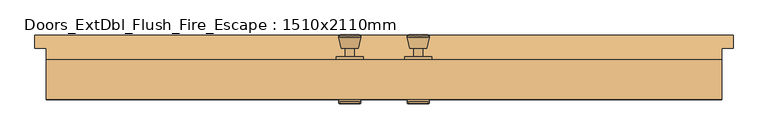
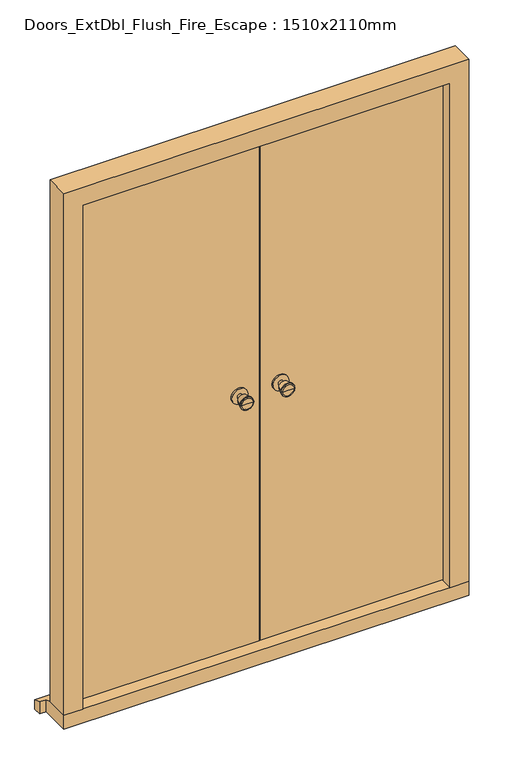
"""IFC4 building model written with IfcOpenShell, lengths in millimetres: door geometry, Doors_ExtDbl_Flush_Fire_Escape : 1510x2110mm."""

from ifc_helpers import new_model, si_unit, point, frame, frame_2d, origin, place, context, project, spatial, polyline, circle_curve, trimmed, segment, composite_curve, outline, extrude, faceted_brep, source, transform, mapped, element, save
from ifc_brep_helpers import plane_surface, cylinder_surface, revolved_surface, advanced_brep


def doors_extdbl_flush_fire_escape_1510x2110mm_f48bbf68(model_context):
    return source(origin(), model_context, "Body", "SolidModel", [
        advanced_brep(
        [(-76.5, 156.0, 1050.0), (-86.5, 156.0, 1050.0), (-66.5, 156.0, 1050.0), (-96.9758676, 205.0, 1050.0), (-76.5, 205.0, 1050.0), (-56.0241324, 205.0, 1050.0), (-101.5, 203.1721319, 1050.0), (-51.5, 203.1721319, 1050.0), (-101.5, 199.7084537, 1050.0), (-51.5, 199.7084537, 1050.0), (-95.136236, 175.0, 1050.0), (-57.863764, 175.0, 1050.0), (-86.5, 175.0, 1050.0), (-66.5, 175.0, 1050.0)],
        [
            (0, 1),
            (1, 2, circle_curve(frame((-76.5, 156.0, 1050.0), z_axis=(0.0, -1.0, 0.0), x_axis=(1.0, 0.0, 0.0)), 10.0)),
            (2, 0),
            (2, 1, circle_curve(frame((-76.5, 156.0, 1050.0), z_axis=(0.0, -1.0, 0.0), x_axis=(1.0, 0.0, 0.0)), 10.0)),
            (3, 4),
            (4, 5),
            (5, 3, circle_curve(frame((-76.5, 205.0, 1050.0), z_axis=(0.0, 1.0, 0.0), x_axis=(1.0, 0.0, 0.0)), 20.4758676)),
            (3, 5, circle_curve(frame((-76.5, 205.0, 1050.0), z_axis=(0.0, 1.0, 0.0), x_axis=(1.0, 0.0, 0.0)), 20.4758676)),
            (6, 3),
            (5, 7),
            (7, 6, circle_curve(frame((-76.5, 203.1721319, 1050.0), z_axis=(0.0, 1.0, 0.0), x_axis=(1.0, 0.0, 0.0)), 25.0)),
            (6, 7, circle_curve(frame((-76.5, 203.1721319, 1050.0), z_axis=(0.0, 1.0, 0.0), x_axis=(1.0, 0.0, 0.0)), 25.0)),
            (8, 6),
            (7, 9),
            (9, 8, circle_curve(frame((-76.5, 199.7084537, 1050.0), z_axis=(0.0, 1.0, 0.0), x_axis=(1.0, 0.0, 0.0)), 25.0)),
            (8, 9, circle_curve(frame((-76.5, 199.7084537, 1050.0), z_axis=(0.0, 1.0, 0.0), x_axis=(1.0, 0.0, 0.0)), 25.0)),
            (10, 8),
            (9, 11),
            (11, 10, circle_curve(frame((-76.5, 175.0, 1050.0), z_axis=(0.0, 1.0, 0.0), x_axis=(1.0, 0.0, 0.0)), 18.636236)),
            (10, 11, circle_curve(frame((-76.5, 175.0, 1050.0), z_axis=(0.0, 1.0, 0.0), x_axis=(1.0, 0.0, 0.0)), 18.636236)),
            (12, 10),
            (11, 13),
            (13, 12, circle_curve(frame((-76.5, 175.0, 1050.0), z_axis=(0.0, 1.0, 0.0), x_axis=(1.0, 0.0, 0.0)), 10.0)),
            (12, 13, circle_curve(frame((-76.5, 175.0, 1050.0), z_axis=(0.0, 1.0, 0.0), x_axis=(1.0, 0.0, 0.0)), 10.0)),
            (1, 12),
            (13, 2),
        ],
        [
            plane_surface(frame((-76.5, 156.0, 1050.0), z_axis=(0.0, -1.0, 0.0), x_axis=(1.0, 0.0, 0.0))),
            plane_surface(frame((-76.5, 205.0, 1050.0), z_axis=(0.0, 1.0, 0.0), x_axis=(1.0, 0.0, 0.0))),
            revolved_surface(polyline([(-56.0241324, 205.0, 1050.0), (-51.5, 203.1721319, 1050.0)]), (-76.5, 156.0, 1050.0), (0.0, -1.0, 0.0)),
            cylinder_surface(frame((-76.5, 156.0, 1050.0), z_axis=(0.0, -1.0, 0.0), x_axis=(1.0, 0.0, 0.0)), 25.0),
            revolved_surface(polyline([(-51.5, 199.7084537, 1050.0), (-57.863764, 175.0, 1050.0)]), (-76.5, 156.0, 1050.0), (0.0, -1.0, 0.0)),
            plane_surface(frame((-76.5, 175.0, 1050.0), z_axis=(0.0, -1.0, 0.0), x_axis=(1.0, 0.0, 0.0))),
            cylinder_surface(frame((-76.5, 156.0, 1050.0), z_axis=(0.0, -1.0, 0.0), x_axis=(1.0, 0.0, 0.0)), 10.0),
        ],
        [
            (0, [[1, 2, 3]]),
            (0, [[-3, 4, -1]]),
            (1, [[5, 6, 7]]),
            (1, [[-6, -5, 8]]),
            (2, [[9, -7, 10, 11]]),
            (2, [[-10, -8, -9, 12]]),
            (3, [[13, -11, 14, 15]]),
            (3, [[-14, -12, -13, 16]]),
            (4, [[17, -15, 18, 19]]),
            (4, [[-18, -16, -17, 20]]),
            (5, [[21, -19, 22, 23]]),
            (5, [[-22, -20, -21, 24]]),
            (6, [[25, -23, 26, -2]]),
            (6, [[-26, -24, -25, -4]]),
        ],
    ),
        extrude(outline(composite_curve([segment(trimmed(circle_curve(frame_2d((1050.0, -76.5)), 30.0), [point((1050.0, -46.5))], [point((1050.0, -106.5))], False, "CARTESIAN"), True, "CONTINUOUS"), segment(trimmed(circle_curve(frame_2d((1050.0, -76.5)), 30.0), [point((1050.0, -106.5))], [point((1050.0, -46.5))], False, "CARTESIAN"), True, "CONTINUOUS")], self_intersect=False)), frame((0.0, 150.0, 0.0), z_axis=(0.0, 1.0, 0.0), x_axis=(0.0, 0.0, 1.0)), (0.0, 0.0, 1.0), 6.0),
        advanced_brep(
        [(-76.5, 100.0, 1050.0), (-66.5, 100.0, 1050.0), (-86.5, 100.0, 1050.0), (-96.9758676, 51.0, 1050.0), (-56.0241324, 51.0, 1050.0), (-76.5, 51.0, 1050.0), (-101.5, 52.8278681, 1050.0), (-51.5, 52.8278681, 1050.0), (-101.5, 56.2915463, 1050.0), (-51.5, 56.2915463, 1050.0), (-95.136236, 81.0, 1050.0), (-57.863764, 81.0, 1050.0), (-86.5, 81.0, 1050.0), (-66.5, 81.0, 1050.0)],
        [
            (0, 1),
            (1, 2, circle_curve(frame((-76.5, 100.0, 1050.0), z_axis=(0.0, 1.0, 0.0), x_axis=(1.0, 0.0, 0.0)), 10.0)),
            (2, 0),
            (2, 1, circle_curve(frame((-76.5, 100.0, 1050.0), z_axis=(0.0, 1.0, 0.0), x_axis=(1.0, 0.0, 0.0)), 10.0)),
            (3, 4, circle_curve(frame((-76.5, 51.0, 1050.0), z_axis=(0.0, -1.0, 0.0), x_axis=(1.0, 0.0, 0.0)), 20.4758676)),
            (4, 5),
            (5, 3),
            (4, 3, circle_curve(frame((-76.5, 51.0, 1050.0), z_axis=(0.0, -1.0, 0.0), x_axis=(1.0, 0.0, 0.0)), 20.4758676)),
            (6, 7, circle_curve(frame((-76.5, 52.8278681, 1050.0), z_axis=(0.0, -1.0, 0.0), x_axis=(1.0, 0.0, 0.0)), 25.0)),
            (7, 4),
            (3, 6),
            (7, 6, circle_curve(frame((-76.5, 52.8278681, 1050.0), z_axis=(0.0, -1.0, 0.0), x_axis=(1.0, 0.0, 0.0)), 25.0)),
            (8, 9, circle_curve(frame((-76.5, 56.2915463, 1050.0), z_axis=(0.0, -1.0, 0.0), x_axis=(1.0, 0.0, 0.0)), 25.0)),
            (9, 7),
            (6, 8),
            (9, 8, circle_curve(frame((-76.5, 56.2915463, 1050.0), z_axis=(0.0, -1.0, 0.0), x_axis=(1.0, 0.0, 0.0)), 25.0)),
            (10, 11, circle_curve(frame((-76.5, 81.0, 1050.0), z_axis=(0.0, -1.0, 0.0), x_axis=(1.0, 0.0, 0.0)), 18.636236)),
            (11, 9),
            (8, 10),
            (11, 10, circle_curve(frame((-76.5, 81.0, 1050.0), z_axis=(0.0, -1.0, 0.0), x_axis=(1.0, 0.0, 0.0)), 18.636236)),
            (12, 13, circle_curve(frame((-76.5, 81.0, 1050.0), z_axis=(0.0, -1.0, 0.0), x_axis=(1.0, 0.0, 0.0)), 10.0)),
            (13, 11),
            (10, 12),
            (13, 12, circle_curve(frame((-76.5, 81.0, 1050.0), z_axis=(0.0, -1.0, 0.0), x_axis=(1.0, 0.0, 0.0)), 10.0)),
            (1, 13),
            (12, 2),
        ],
        [
            plane_surface(frame((-76.5, 100.0, 1050.0), z_axis=(0.0, 1.0, 0.0), x_axis=(1.0, 0.0, 0.0))),
            plane_surface(frame((-76.5, 51.0, 1050.0), z_axis=(0.0, -1.0, 0.0), x_axis=(1.0, 0.0, 0.0))),
            revolved_surface(polyline([(-56.0241324, 51.0, 1050.0), (-51.5, 52.8278681, 1050.0)]), (-76.5, 100.0, 1050.0), (0.0, 1.0, 0.0)),
            cylinder_surface(frame((-76.5, 100.0, 1050.0), z_axis=(0.0, 1.0, 0.0), x_axis=(1.0, 0.0, 0.0)), 25.0),
            revolved_surface(polyline([(-51.5, 56.2915463, 1050.0), (-57.863764, 81.0, 1050.0)]), (-76.5, 100.0, 1050.0), (0.0, 1.0, 0.0)),
            plane_surface(frame((-76.5, 81.0, 1050.0), z_axis=(0.0, 1.0, 0.0), x_axis=(1.0, 0.0, 0.0))),
            cylinder_surface(frame((-76.5, 100.0, 1050.0), z_axis=(0.0, 1.0, 0.0), x_axis=(1.0, 0.0, 0.0)), 10.0),
        ],
        [
            (0, [[1, 2, 3]]),
            (0, [[-3, 4, -1]]),
            (1, [[5, 6, 7]]),
            (1, [[8, -7, -6]]),
            (2, [[9, 10, -5, 11]]),
            (2, [[12, -11, -8, -10]]),
            (3, [[13, 14, -9, 15]]),
            (3, [[16, -15, -12, -14]]),
            (4, [[17, 18, -13, 19]]),
            (4, [[20, -19, -16, -18]]),
            (5, [[21, 22, -17, 23]]),
            (5, [[24, -23, -20, -22]]),
            (6, [[-2, 25, -21, 26]]),
            (6, [[-4, -26, -24, -25]]),
        ],
    ),
        extrude(outline(composite_curve([segment(trimmed(circle_curve(frame_2d((1050.0, -76.5)), 30.0), [point((1050.0, -46.5))], [point((1050.0, -106.5))], False, "CARTESIAN"), True, "CONTINUOUS"), segment(trimmed(circle_curve(frame_2d((1050.0, -76.5)), 30.0), [point((1050.0, -106.5))], [point((1050.0, -46.5))], False, "CARTESIAN"), True, "CONTINUOUS")], self_intersect=False)), frame((0.0, 100.0, 0.0), z_axis=(0.0, 1.0, 0.0), x_axis=(0.0, 0.0, 1.0)), (0.0, 0.0, 1.0), 6.0),
        advanced_brep(
        [(76.5, 156.0, 1050.0), (66.5, 156.0, 1050.0), (86.5, 156.0, 1050.0), (96.9758676, 205.0, 1050.0), (56.0241324, 205.0, 1050.0), (76.5, 205.0, 1050.0), (101.5, 203.1721319, 1050.0), (51.5, 203.1721319, 1050.0), (101.5, 199.7084537, 1050.0), (51.5, 199.7084537, 1050.0), (95.136236, 175.0, 1050.0), (57.863764, 175.0, 1050.0), (86.5, 175.0, 1050.0), (66.5, 175.0, 1050.0)],
        [
            (0, 1),
            (1, 2, circle_curve(frame((76.5, 156.0, 1050.0), z_axis=(0.0, -1.0, 0.0), x_axis=(-1.0, 0.0, 0.0)), 10.0)),
            (2, 0),
            (2, 1, circle_curve(frame((76.5, 156.0, 1050.0), z_axis=(0.0, -1.0, 0.0), x_axis=(-1.0, 0.0, 0.0)), 10.0)),
            (3, 4, circle_curve(frame((76.5, 205.0, 1050.0), z_axis=(0.0, 1.0, 0.0), x_axis=(-1.0, 0.0, 0.0)), 20.4758676)),
            (4, 5),
            (5, 3),
            (4, 3, circle_curve(frame((76.5, 205.0, 1050.0), z_axis=(0.0, 1.0, 0.0), x_axis=(-1.0, 0.0, 0.0)), 20.4758676)),
            (6, 7, circle_curve(frame((76.5, 203.1721319, 1050.0), z_axis=(0.0, 1.0, 0.0), x_axis=(-1.0, 0.0, 0.0)), 25.0)),
            (7, 4),
            (3, 6),
            (7, 6, circle_curve(frame((76.5, 203.1721319, 1050.0), z_axis=(0.0, 1.0, 0.0), x_axis=(-1.0, 0.0, 0.0)), 25.0)),
            (8, 9, circle_curve(frame((76.5, 199.7084537, 1050.0), z_axis=(0.0, 1.0, 0.0), x_axis=(-1.0, 0.0, 0.0)), 25.0)),
            (9, 7),
            (6, 8),
            (9, 8, circle_curve(frame((76.5, 199.7084537, 1050.0), z_axis=(0.0, 1.0, 0.0), x_axis=(-1.0, 0.0, 0.0)), 25.0)),
            (10, 11, circle_curve(frame((76.5, 175.0, 1050.0), z_axis=(0.0, 1.0, 0.0), x_axis=(-1.0, 0.0, 0.0)), 18.636236)),
            (11, 9),
            (8, 10),
            (11, 10, circle_curve(frame((76.5, 175.0, 1050.0), z_axis=(0.0, 1.0, 0.0), x_axis=(-1.0, 0.0, 0.0)), 18.636236)),
            (12, 13, circle_curve(frame((76.5, 175.0, 1050.0), z_axis=(0.0, 1.0, 0.0), x_axis=(-1.0, 0.0, 0.0)), 10.0)),
            (13, 11),
            (10, 12),
            (13, 12, circle_curve(frame((76.5, 175.0, 1050.0), z_axis=(0.0, 1.0, 0.0), x_axis=(-1.0, 0.0, 0.0)), 10.0)),
            (1, 13),
            (12, 2),
        ],
        [
            plane_surface(frame((76.5, 156.0, 1050.0), z_axis=(0.0, -1.0, 0.0), x_axis=(-1.0, 0.0, 0.0))),
            plane_surface(frame((76.5, 205.0, 1050.0), z_axis=(0.0, 1.0, 0.0), x_axis=(-1.0, 0.0, 0.0))),
            revolved_surface(polyline([(56.0241324, 205.0, 1050.0), (51.5, 203.1721319, 1050.0)]), (76.5, 156.0, 1050.0), (0.0, -1.0, 0.0)),
            cylinder_surface(frame((76.5, 156.0, 1050.0), z_axis=(0.0, -1.0, 0.0), x_axis=(-1.0, 0.0, 0.0)), 25.0),
            revolved_surface(polyline([(51.5, 199.7084537, 1050.0), (57.863764, 175.0, 1050.0)]), (76.5, 156.0, 1050.0), (0.0, -1.0, 0.0)),
            plane_surface(frame((76.5, 175.0, 1050.0), z_axis=(0.0, -1.0, 0.0), x_axis=(-1.0, 0.0, 0.0))),
            cylinder_surface(frame((76.5, 156.0, 1050.0), z_axis=(0.0, -1.0, 0.0), x_axis=(-1.0, 0.0, 0.0)), 10.0),
        ],
        [
            (0, [[1, 2, 3]]),
            (0, [[-3, 4, -1]]),
            (1, [[5, 6, 7]]),
            (1, [[8, -7, -6]]),
            (2, [[9, 10, -5, 11]]),
            (2, [[12, -11, -8, -10]]),
            (3, [[13, 14, -9, 15]]),
            (3, [[16, -15, -12, -14]]),
            (4, [[17, 18, -13, 19]]),
            (4, [[20, -19, -16, -18]]),
            (5, [[21, 22, -17, 23]]),
            (5, [[24, -23, -20, -22]]),
            (6, [[-2, 25, -21, 26]]),
            (6, [[-4, -26, -24, -25]]),
        ],
    ),
        extrude(outline(composite_curve([segment(trimmed(circle_curve(frame_2d((1050.0, 76.5)), 30.0), [point((1050.0, 46.5))], [point((1050.0, 106.5))], False, "CARTESIAN"), True, "CONTINUOUS"), segment(trimmed(circle_curve(frame_2d((1050.0, 76.5)), 30.0), [point((1050.0, 106.5))], [point((1050.0, 46.5))], False, "CARTESIAN"), True, "CONTINUOUS")], self_intersect=False)), frame((0.0, 150.0, 0.0), z_axis=(0.0, 1.0, 0.0), x_axis=(0.0, 0.0, 1.0)), (0.0, 0.0, 1.0), 6.0),
        advanced_brep(
        [(76.5, 100.0, 1050.0), (86.5, 100.0, 1050.0), (66.5, 100.0, 1050.0), (96.9758676, 51.0, 1050.0), (76.5, 51.0, 1050.0), (56.0241324, 51.0, 1050.0), (101.5, 52.8278681, 1050.0), (51.5, 52.8278681, 1050.0), (101.5, 56.2915463, 1050.0), (51.5, 56.2915463, 1050.0), (95.136236, 81.0, 1050.0), (57.863764, 81.0, 1050.0), (86.5, 81.0, 1050.0), (66.5, 81.0, 1050.0)],
        [
            (0, 1),
            (1, 2, circle_curve(frame((76.5, 100.0, 1050.0), z_axis=(0.0, 1.0, 0.0), x_axis=(-1.0, 0.0, 0.0)), 10.0)),
            (2, 0),
            (2, 1, circle_curve(frame((76.5, 100.0, 1050.0), z_axis=(0.0, 1.0, 0.0), x_axis=(-1.0, 0.0, 0.0)), 10.0)),
            (3, 4),
            (4, 5),
            (5, 3, circle_curve(frame((76.5, 51.0, 1050.0), z_axis=(0.0, -1.0, 0.0), x_axis=(-1.0, 0.0, 0.0)), 20.4758676)),
            (3, 5, circle_curve(frame((76.5, 51.0, 1050.0), z_axis=(0.0, -1.0, 0.0), x_axis=(-1.0, 0.0, 0.0)), 20.4758676)),
            (6, 3),
            (5, 7),
            (7, 6, circle_curve(frame((76.5, 52.8278681, 1050.0), z_axis=(0.0, -1.0, 0.0), x_axis=(-1.0, 0.0, 0.0)), 25.0)),
            (6, 7, circle_curve(frame((76.5, 52.8278681, 1050.0), z_axis=(0.0, -1.0, 0.0), x_axis=(-1.0, 0.0, 0.0)), 25.0)),
            (8, 6),
            (7, 9),
            (9, 8, circle_curve(frame((76.5, 56.2915463, 1050.0), z_axis=(0.0, -1.0, 0.0), x_axis=(-1.0, 0.0, 0.0)), 25.0)),
            (8, 9, circle_curve(frame((76.5, 56.2915463, 1050.0), z_axis=(0.0, -1.0, 0.0), x_axis=(-1.0, 0.0, 0.0)), 25.0)),
            (10, 8),
            (9, 11),
            (11, 10, circle_curve(frame((76.5, 81.0, 1050.0), z_axis=(0.0, -1.0, 0.0), x_axis=(-1.0, 0.0, 0.0)), 18.636236)),
            (10, 11, circle_curve(frame((76.5, 81.0, 1050.0), z_axis=(0.0, -1.0, 0.0), x_axis=(-1.0, 0.0, 0.0)), 18.636236)),
            (12, 10),
            (11, 13),
            (13, 12, circle_curve(frame((76.5, 81.0, 1050.0), z_axis=(0.0, -1.0, 0.0), x_axis=(-1.0, 0.0, 0.0)), 10.0)),
            (12, 13, circle_curve(frame((76.5, 81.0, 1050.0), z_axis=(0.0, -1.0, 0.0), x_axis=(-1.0, 0.0, 0.0)), 10.0)),
            (1, 12),
            (13, 2),
        ],
        [
            plane_surface(frame((76.5, 100.0, 1050.0), z_axis=(0.0, 1.0, 0.0), x_axis=(-1.0, 0.0, 0.0))),
            plane_surface(frame((76.5, 51.0, 1050.0), z_axis=(0.0, -1.0, 0.0), x_axis=(-1.0, 0.0, 0.0))),
            revolved_surface(polyline([(56.0241324, 51.0, 1050.0), (51.5, 52.8278681, 1050.0)]), (76.5, 100.0, 1050.0), (0.0, 1.0, 0.0)),
            cylinder_surface(frame((76.5, 100.0, 1050.0), z_axis=(0.0, 1.0, 0.0), x_axis=(-1.0, 0.0, 0.0)), 25.0),
            revolved_surface(polyline([(51.5, 56.2915463, 1050.0), (57.863764, 81.0, 1050.0)]), (76.5, 100.0, 1050.0), (0.0, 1.0, 0.0)),
            plane_surface(frame((76.5, 81.0, 1050.0), z_axis=(0.0, 1.0, 0.0), x_axis=(-1.0, 0.0, 0.0))),
            cylinder_surface(frame((76.5, 100.0, 1050.0), z_axis=(0.0, 1.0, 0.0), x_axis=(-1.0, 0.0, 0.0)), 10.0),
        ],
        [
            (0, [[1, 2, 3]]),
            (0, [[-3, 4, -1]]),
            (1, [[5, 6, 7]]),
            (1, [[-6, -5, 8]]),
            (2, [[9, -7, 10, 11]]),
            (2, [[-10, -8, -9, 12]]),
            (3, [[13, -11, 14, 15]]),
            (3, [[-14, -12, -13, 16]]),
            (4, [[17, -15, 18, 19]]),
            (4, [[-18, -16, -17, 20]]),
            (5, [[21, -19, 22, 23]]),
            (5, [[-22, -20, -21, 24]]),
            (6, [[25, -23, 26, -2]]),
            (6, [[-26, -24, -25, -4]]),
        ],
    ),
        extrude(outline(composite_curve([segment(trimmed(circle_curve(frame_2d((1050.0, 76.5)), 30.0), [point((1050.0, 46.5))], [point((1050.0, 106.5))], False, "CARTESIAN"), True, "CONTINUOUS"), segment(trimmed(circle_curve(frame_2d((1050.0, 76.5)), 30.0), [point((1050.0, 106.5))], [point((1050.0, 46.5))], False, "CARTESIAN"), True, "CONTINUOUS")], self_intersect=False)), frame((0.0, 100.0, 0.0), z_axis=(0.0, 1.0, 0.0), x_axis=(0.0, 0.0, 1.0)), (0.0, 0.0, 1.0), 6.0),
        faceted_brep([(706.5, 150.0, 54.5), (755.0, 150.0, 54.5), (755.0, 61.0, 54.5), (684.5, 61.0, 54.5), (684.5, 103.0, 54.5), (706.5, 103.0, 54.5), (706.5, 150.0, 2061.5), (-706.5, 150.0, 2061.5), (-706.5, 150.0, 54.5), (-755.0, 150.0, 54.5), (-755.0, 150.0, 2110.0), (755.0, 150.0, 2110.0), (755.0, 61.0, 2110.0), (-755.0, 61.0, 2110.0), (-755.0, 61.0, 54.5), (-684.5, 61.0, 54.5), (-684.5, 61.0, 2039.5), (684.5, 61.0, 2039.5), (684.5, 103.0, 2039.5), (-684.5, 103.0, 2039.5), (-684.5, 103.0, 54.5), (-706.5, 103.0, 54.5), (-706.5, 103.0, 2061.5), (706.5, 103.0, 2061.5)], [[[0, 1, 2, 3, 4, 5]], [[1, 0, 6, 7, 8, 9, 10, 11]], [[2, 1, 11, 12]], [[3, 2, 12, 13, 14, 15, 16, 17]], [[4, 3, 17, 18]], [[5, 4, 18, 19, 20, 21, 22, 23]], [[0, 5, 23, 6]], [[7, 22, 21, 8]], [[8, 21, 20, 15, 14, 9]], [[13, 10, 9, 14]], [[19, 16, 15, 20]], [[12, 11, 10, 13]], [[18, 17, 16, 19]], [[6, 23, 22, 7]]]),
        extrude(outline(polyline([(1.5, 150.0), (703.5, 150.0), (703.5, 106.0), (1.5, 106.0), (1.5, 150.0)])), frame((0.0, 0.0, 58.5), z_axis=(0.0, 0.0, 1.0), x_axis=(1.0, 0.0, 0.0)), (0.0, 0.0, 1.0), 2000.0),
        extrude(outline(polyline([(-703.5, 150.0), (-1.5, 150.0), (-1.5, 106.0), (-703.5, 106.0), (-703.5, 150.0)])), frame((0.0, 0.0, 58.5), z_axis=(0.0, 0.0, 1.0), x_axis=(1.0, 0.0, 0.0)), (0.0, 0.0, 1.0), 2000.0),
        faceted_brep([(780.0, 205.0, 0.0), (780.0, 205.0, 38.5947221), (780.0, 175.0, 47.2703282), (780.0, 175.0, 0.0), (-780.0, 205.0, 38.5947221), (-780.0, 205.0, 0.0), (-780.0, 175.0, 0.0), (-780.0, 175.0, 47.2703282), (755.0, 175.0, 0.0), (755.0, 61.0, 0.0), (-755.0, 61.0, 0.0), (-755.0, 175.0, 0.0), (-755.0, 175.0, 47.2703282), (-755.0, 150.0, 54.5), (755.0, 150.0, 54.5), (755.0, 175.0, 47.2703282), (-755.0, 61.0, 54.5), (755.0, 61.0, 54.5)], [[[0, 1, 2, 3]], [[4, 5, 6, 7]], [[5, 0, 3, 8, 9, 10, 11, 6]], [[1, 0, 5, 4]], [[1, 4, 7, 12, 13, 14, 15, 2]], [[13, 16, 17, 14]], [[16, 10, 9, 17]], [[12, 11, 10, 16, 13]], [[11, 12, 7, 6]], [[8, 15, 14, 17, 9]], [[15, 8, 3, 2]]]),
    ])


if __name__ == "__main__":
    model = new_model("IFC4")
    model_context = context("Model", 3, world=origin())
    ifc_project = project(units=[si_unit("LENGTHUNIT", "METRE", prefix="MILLI")], contexts=[model_context])
    site = spatial("IfcSite", under=ifc_project)
    building = spatial("IfcBuilding", under=site)
    placement = place(None, origin())
    doors_extdbl_flush_fire_escape_1510x2110mm_shape = doors_extdbl_flush_fire_escape_1510x2110mm_f48bbf68(model_context)
    element("IfcDoor", 1, ObjectType="Doors_ExtDbl_Flush_Fire_Escape : 1510x2110mm", at=placement, inside=building, context=model_context, shape_type="MappedRepresentation", body=[
        mapped(doors_extdbl_flush_fire_escape_1510x2110mm_shape, transform((0.0, 0.0, 0.0), x_axis=(1.0, 0.0, 0.0), y_axis=(0.0, 1.0, 0.0), z_axis=(0.0, 0.0, 1.0))),
    ])
    save(model, "model.ifc")

# Revit data of these elements
# Type "Doors_ExtDbl_Flush_Fire_Escape : 1510x2110mm"
#   Type Mark = "50"
#   Type Comments = "External Double"
#   Operation = "DoubleDoorSingleSwing"
#   Construction Type Id = "MDOOR"
#   Keynote = "L20"
#   Description = "External Opening Double Doors"
#   Analytic Construction = "Metal"
#   Wrap Layers (Ext) from Ext = 102.5 mm
#   Wrap Layers (Int) from Ext = 177.5 mm
#   Thickness = 44 mm
#   Rough Width = 1510 mm
#   Rough Height = 2110 mm
#   O/A Frame Width = 64 mm
#   Heat Transfer Coefficient (U) = 3.7021 W/(m²·K)
#   Handle Z Distance = 1050 mm
#   FrameWidth = 42 mm
#   FrameOffset - External = 25 mm
#   FrameDepth = 89 mm
#   Door Panel Width = 702 mm
#   Door Panel Thickness = 44 mm
#   Door Panel Height = 2000 mm
#   Cill Thickness = 54.5 mm
#   Cill Projection = 30 mm
#   Handle X Distance = 75 mm
#   Height = 2110 mm
#   Structural Tolerance = 6.5 mm
#   Tolerance = 3 mm
#   Undercut = 4 mm
#   Width = 1510 mm
#   Cill Extension = 25 mm
#   Cavity Closer Width = 50 mm
#   Cavity Closer Offset from Ext = 102.5 mm
#   Cavity Closer Depth = 85 mm
#   Vis - Ironmongery = yes
#   Vis - Cavity Closers = yes
#   Define Thermal Properties by = 1
#   Function = 1
#   Material Door = Door - Panel
#   Material Frame = Door - Frame/Mullion
#   Material Ironmongery = Door - Handle
#   Visual Light Transmittance = 0
#   Solar Heat Gain Coefficient = 0
#   Wall Closure = (empty or 0)
# Element 1 (IfcDoor, "Doors_ExtDbl_Flush_Fire_Escape : 1510x2110mm")
#   Materials on its faces: "Door - Handle", "Door - Frame/Mullion", "Door - Panel"
# Materials
#   "Door - Panel": class "Wood", colour RGB 210 159 95, transparency 0, Keynote = "L20", Cost = 0
#   "Door - Frame/Mullion": class "Wood", colour RGB 212 179 113, transparency 0, Keynote = "L20", Cost = 0
#   "Door - Handle": class "Miscellaneous", colour RGB 0 0 0, transparency 0, Keynote = "P21", Cost = 0
